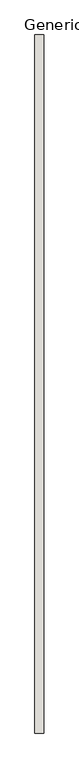
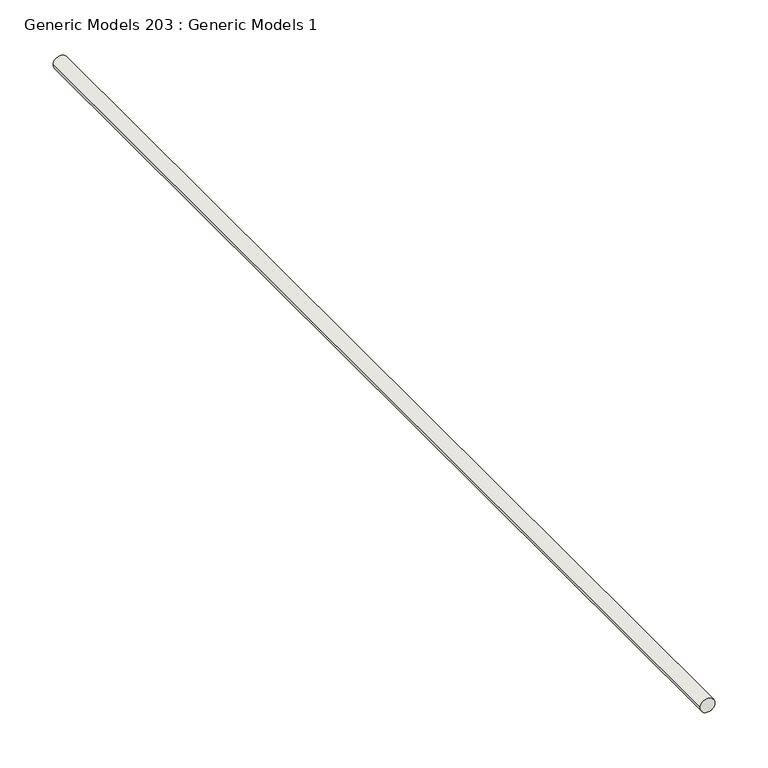
"""IFC4 building model written with IfcOpenShell, lengths in millimetres: wall geometry, Generic Models 203 : Generic Models 1."""

from ifc_helpers import new_model, si_unit, point, frame, frame_2d, origin, place, context, project, spatial, circle_curve, trimmed, segment, composite_curve, outline, extrude, source, transform, mapped, element, save


def generic_models_203_generic_models_1_7f2b1a48(model_context):
    return source(origin(), model_context, "Body", "SweptSolid", [
        extrude(outline(composite_curve([segment(trimmed(circle_curve(frame_2d((2275.8814234, 748109.175479)), 7.9375), [point((2275.8814234, 748117.112979))], [point((2275.8814234, 748101.237979))], False, "CARTESIAN"), True, "CONTINUOUS"), segment(trimmed(circle_curve(frame_2d((2275.8814234, 748109.175479)), 7.9375), [point((2275.8814234, 748101.237979))], [point((2275.8814234, 748117.112979))], False, "CARTESIAN"), True, "CONTINUOUS")], self_intersect=False)), frame((0.0, 76.2, 0.0), z_axis=(0.0, 1.0, 0.0), x_axis=(0.0, 0.0, 1.0)), (0.0, 0.0, 1.0), 1219.2),
    ])


if __name__ == "__main__":
    model = new_model("IFC4")
    model_context = context("Model", 3, world=origin())
    ifc_project = project(units=[si_unit("LENGTHUNIT", "METRE", prefix="MILLI")], contexts=[model_context])
    site = spatial("IfcSite", under=ifc_project)
    building = spatial("IfcBuilding", under=site)
    placement = place(None, origin())
    generic_models_203_generic_models_1_shape = generic_models_203_generic_models_1_7f2b1a48(model_context)
    element("IfcWall", 1, ObjectType="Generic Models 203 : Generic Models 1", at=placement, inside=building, context=model_context, shape_type="MappedRepresentation", body=[
        mapped(generic_models_203_generic_models_1_shape, transform((0.0, 0.0, 0.0), x_axis=(1.0, 0.0, 0.0), y_axis=(0.0, 1.0, 0.0), z_axis=(0.0, 0.0, 1.0))),
    ])
    save(model, "model.ifc")

# Revit data of these elements
# Element 1 (IfcWall, "Generic Models 203 : Generic Models 1")
#   Materials on its faces: "(2) #5's"
# Materials
#   "(2) #5's": class "Generic", colour RGB 255 255 255, transparency 0, Cost = 0
